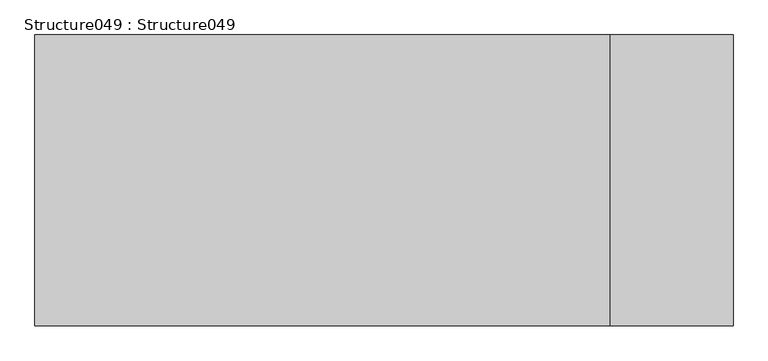
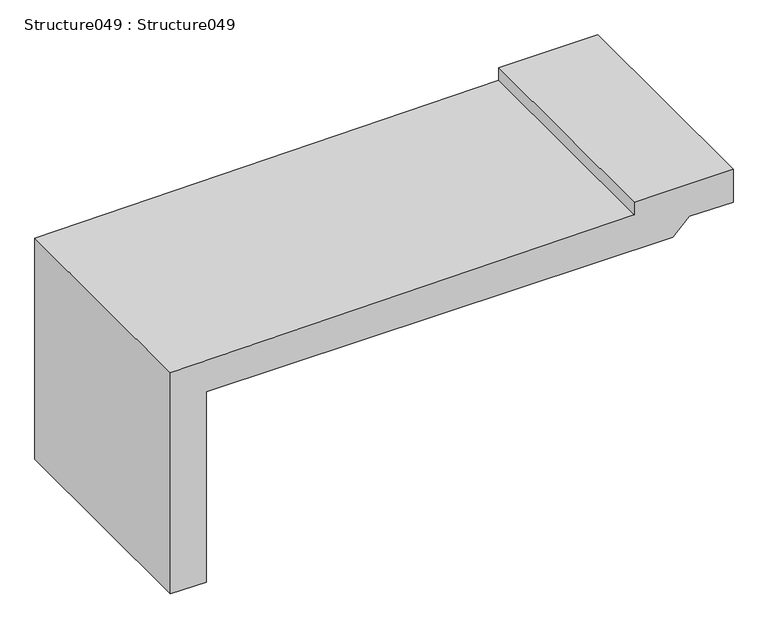
"""IFC4 building model written with IfcOpenShell, lengths in millimetres: proxy geometry, Structure049 : Structure049."""

from ifc_helpers import new_model, si_unit, frame, origin, place, context, project, spatial, polyline, outline, extrude, source, transform, mapped, element, save


def structure049_structure049_81cae09d(model_context):
    return source(origin(), model_context, "Body", "SweptSolid", [
        extrude(outline(polyline([(34435.796, -5752.3008907), (36150.296, -5752.3008907), (36150.296, -1775.3101807), (36288.4960937, -1630.9492188), (36288.4960937, -1259.2199707), (36582.096, -1259.2199707), (36582.096, -2103.1864422), (36467.796, -2103.1864422), (36429.696, -6057.1008907), (34435.796, -6057.1008907), (34435.796, -5752.3008907)])), frame((0.0, -1052.8906574, 0.0), z_axis=(0.0, 1.0, 0.0), x_axis=(0.0, 0.0, 1.0)), (0.0, 0.0, 1.0), 2000.0),
    ])


if __name__ == "__main__":
    model = new_model("IFC4")
    model_context = context("Model", 3, world=origin())
    ifc_project = project(units=[si_unit("LENGTHUNIT", "METRE", prefix="MILLI")], contexts=[model_context])
    site = spatial("IfcSite", under=ifc_project)
    building = spatial("IfcBuilding", under=site)
    placement = place(None, origin())
    structure049_structure049_shape = structure049_structure049_81cae09d(model_context)
    element("IfcBuildingElementProxy", 1, Name="Structure049 : Structure049", ObjectType="Structure049 : Structure049", at=placement, inside=building, context=model_context, shape_type="MappedRepresentation", body=[
        mapped(structure049_structure049_shape, transform((0.0, 0.0, 0.0), x_axis=(1.0, 0.0, 0.0), y_axis=(0.0, 1.0, 0.0), z_axis=(0.0, 0.0, 1.0))),
    ])
    save(model, "model.ifc")

# Revit data of these elements
# Type "Structure049 : Structure049"
#   NameOverride = "Structure049"
# Element 1 (IfcBuildingElementProxy, "Structure049 : Structure049")
#   Materials on its faces: "4\" CONCRETE SLAB - SEE CIVIL DWGS"
# Materials
#   "4\" CONCRETE SLAB - SEE CIVIL DWGS": class "Unassigned", colour RGB 128 128 128, transparency 0, Cost = 0
